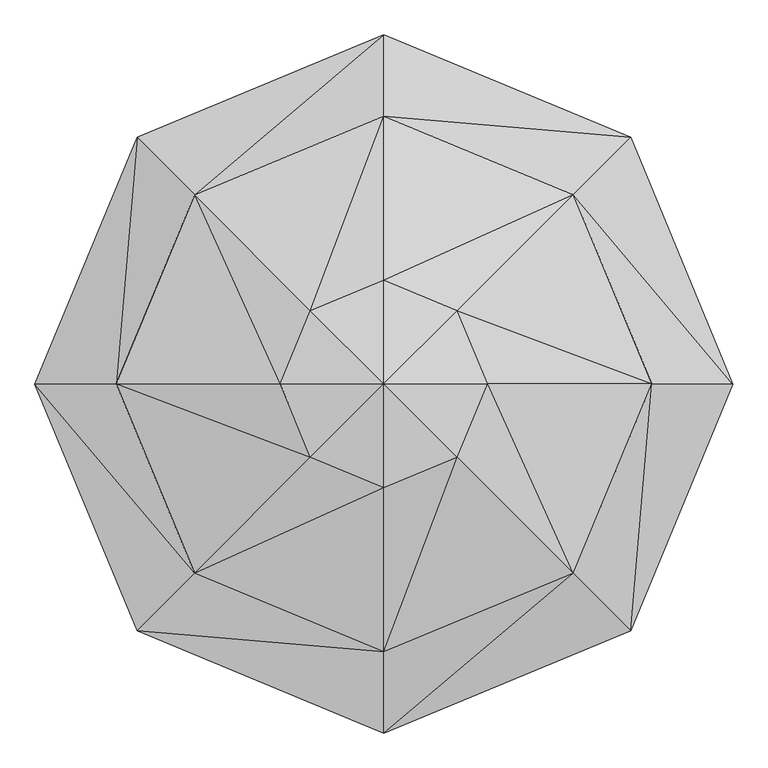
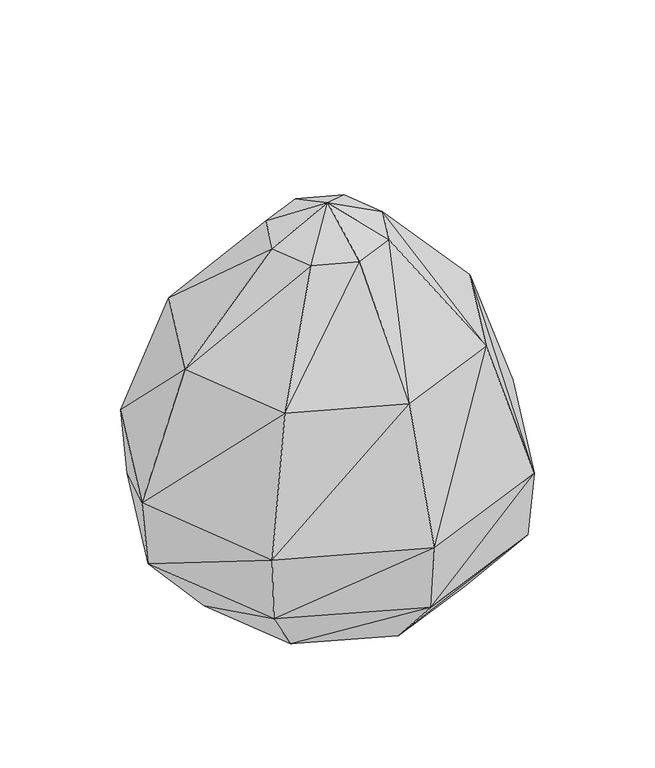
"""IFC4 building model written with IfcOpenShell, lengths in millimetres: geographic element geometry, Enscape AssetDefinition - Bush 014 English Laurel : Enscape AssetDefinition - Bush 014 English Laurel."""

from ifc_helpers import new_model, si_unit, origin, place, context, project, spatial, faceted_brep, source, transform, mapped, element, save


def geographic_element_b2445dd4(model_context):
    return source(origin(), model_context, "Body", "Brep", [
        faceted_brep([(560.1119995, 563.4410977, 288.7996435), (543.1887507, 0.0, 2.2790367), (383.1171691, 386.447221, 2.2790367), (793.4967279, 0.0, 288.7996435), (383.1181526, -386.4462376, 2.2790367), (578.8843036, 582.2134018, 582.6673508), (-3.3290535, 796.8257666, 288.7996435), (-3.3290535, 823.3732581, 582.6673508), (820.0441599, 0.0, 582.6673508), (560.1119995, -563.4410977, 288.7996435), (-3.3290535, -546.5177894, 2.2790367), (-389.7752464, -386.447221, 2.2790367), (-3.3290535, -796.8257666, 288.7996435), (578.8843036, -582.2123289, 582.6673508), (443.4561133, 446.7851818, 1142.8493261), (628.5211444, 0.0, 1142.8493261), (-3.3290535, -823.3732581, 582.6673508), (443.4561133, -446.7851818, 1142.8493261), (-566.7691231, -563.4410977, 288.7996435), (-585.5414271, -582.2134018, 582.6673508), (-3.3290535, -631.8501234, 1142.8493261), (169.9197292, -173.2487828, 1572.6302862), (241.6819036, 0.0, 1572.6302862), (169.9197292, 173.2487828, 1572.6302862), (-3.3290535, 0.0, 1701.1973858), (-3.3290535, -245.0109422, 1572.6302862), (-450.1142502, -446.7851818, 1142.8493261), (-176.5778363, -173.2487828, 1572.6302862), (-3.3290535, 245.0109422, 1572.6302862), (-176.5778363, 173.2487828, 1572.6302862), (-248.3399808, 0.0, 1572.6302862), (-3.3290535, 631.8501234, 1142.8493261), (-450.1142502, 446.7851818, 1142.8493261), (-635.1792216, 0.0, 1142.8493261), (-585.5423808, 582.2134018, 582.6673508), (-826.7022967, 0.0, 582.6673508), (-566.7701364, 563.4410977, 288.7996435), (-800.1548648, 0.0, 288.7996435), (-3.3290535, 546.5177894, 2.2790367), (-389.7752464, 386.4462376, 2.2790367), (-549.846828, 0.0, 2.2790367)], [[[0, 1, 2]], [[1, 0, 3]], [[3, 4, 1]], [[2, 1, 4]], [[5, 3, 0]], [[2, 6, 0]], [[7, 0, 6]], [[0, 7, 5]], [[3, 5, 8]], [[4, 3, 9]], [[8, 9, 3]], [[9, 10, 4]], [[11, 4, 10]], [[2, 4, 11]], [[10, 9, 12]], [[13, 12, 9]], [[9, 8, 13]], [[14, 8, 5]], [[8, 14, 15]], [[15, 13, 8]], [[12, 13, 16]], [[17, 16, 13]], [[13, 15, 17]], [[12, 11, 10]], [[11, 12, 18]], [[16, 18, 12]], [[18, 16, 19]], [[20, 19, 16]], [[16, 17, 20]], [[21, 20, 17]], [[22, 17, 15]], [[17, 22, 21]], [[23, 15, 14]], [[15, 23, 22]], [[24, 22, 23]], [[24, 21, 22]], [[20, 21, 25]], [[24, 25, 21]], [[19, 20, 26]], [[25, 26, 20]], [[26, 25, 27]], [[24, 27, 25]], [[24, 23, 28]], [[24, 28, 29]], [[24, 29, 30]], [[24, 30, 27]], [[14, 28, 23]], [[28, 14, 31]], [[31, 29, 28]], [[29, 31, 32]], [[32, 30, 29]], [[30, 32, 33]], [[33, 27, 30]], [[27, 33, 26]], [[33, 34, 35]], [[34, 33, 32]], [[35, 26, 33]], [[32, 7, 34]], [[7, 32, 31]], [[31, 5, 7]], [[5, 31, 14]], [[6, 34, 7]], [[34, 6, 36]], [[36, 35, 34]], [[35, 36, 37]], [[37, 19, 35]], [[26, 35, 19]], [[36, 38, 39]], [[38, 36, 6]], [[39, 37, 36]], [[6, 2, 38]], [[2, 39, 38]], [[37, 39, 40]], [[39, 11, 40]], [[2, 11, 39]], [[40, 18, 37]], [[19, 37, 18]], [[18, 40, 11]]]),
    ])


if __name__ == "__main__":
    model = new_model("IFC4")
    model_context = context("Model", 3, world=origin())
    ifc_project = project(units=[si_unit("LENGTHUNIT", "METRE", prefix="MILLI")], contexts=[model_context])
    site = spatial("IfcSite", under=ifc_project)
    building = spatial("IfcBuilding", under=site)
    placement = place(None, origin())
    geographic_element_shape = geographic_element_b2445dd4(model_context)
    element("IfcGeographicElement", 1, ObjectType="Enscape AssetDefinition - Bush 014 English Laurel : Enscape AssetDefinition - Bush 014 English Laurel", at=placement, inside=building, context=model_context, shape_type="MappedRepresentation", body=[
        mapped(geographic_element_shape, transform((0.0, 0.0, 0.0), x_axis=(1.0, 0.0, 0.0), y_axis=(0.0, 1.0, 0.0), z_axis=(0.0, 0.0, 1.0))),
    ])
    save(model, "model.ifc")

# Revit data of these elements
# Type "Enscape AssetDefinition - Bush 014 English Laurel : Enscape AssetDefinition - Bush 014 English Laurel"
#   EnscapeAssetSource = "REMOTE"
#   EnscapeAssetId = "34d54a6f-f222-406d-adfd-37700d9ff281"
#   Height = 1.701197 m
#   EnscapeNativeAssetHeight = 1.701197 m
#   Default Elevation = 0
